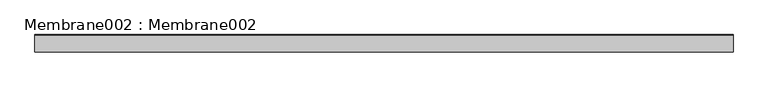
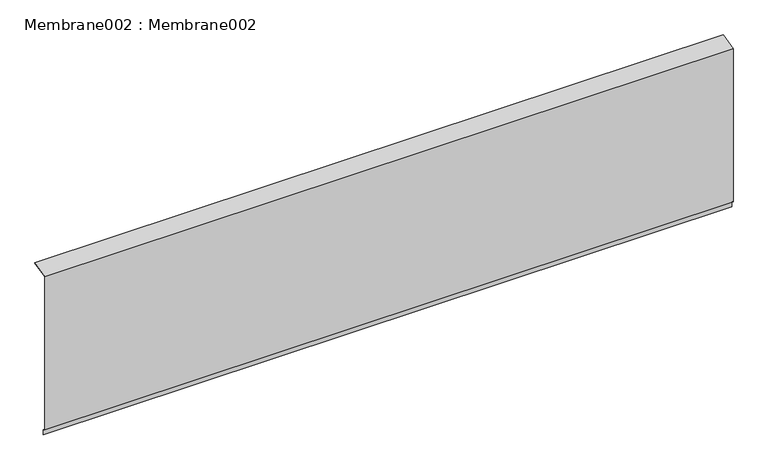
"""IFC4 building model written with IfcOpenShell, lengths in millimetres: proxy geometry, Membrane002 : Membrane002."""

from ifc_helpers import new_model, si_unit, frame, origin, place, context, project, spatial, polyline, outline, extrude, source, transform, mapped, element, save


def membrane002_membrane002_5acc3b50(model_context):
    return source(origin(), model_context, "Body", "SweptSolid", [
        extrude(outline(polyline([(10487.9371885, 43422.3848589), (10439.3258229, 43410.2922698), (10439.3258229, 42942.6633437), (10446.7216797, 42936.3899062), (10446.7216797, 42922.2460937), (10445.2216797, 42922.2460937), (10445.2216797, 42935.6953125), (10437.8258229, 42941.96875), (10437.8258229, 43411.4648437), (10487.5750834, 43423.8404962), (10487.9371885, 43422.3848589)])), frame((3694.2883192, 0.0, 0.0), z_axis=(1.0, 0.0, 0.0), x_axis=(0.0, 1.0, 0.0)), (0.0, 0.0, 1.0), 2000.0),
    ])


if __name__ == "__main__":
    model = new_model("IFC4")
    model_context = context("Model", 3, world=origin())
    ifc_project = project(units=[si_unit("LENGTHUNIT", "METRE", prefix="MILLI")], contexts=[model_context])
    site = spatial("IfcSite", under=ifc_project)
    building = spatial("IfcBuilding", under=site)
    placement = place(None, origin())
    membrane002_membrane002_shape = membrane002_membrane002_5acc3b50(model_context)
    element("IfcBuildingElementProxy", 1, Name="Membrane002 : Membrane002", ObjectType="Membrane002 : Membrane002", at=placement, inside=building, context=model_context, shape_type="MappedRepresentation", body=[
        mapped(membrane002_membrane002_shape, transform((0.0, 0.0, 0.0), x_axis=(1.0, 0.0, 0.0), y_axis=(0.0, 1.0, 0.0), z_axis=(0.0, 0.0, 1.0))),
    ])
    save(model, "model.ifc")

# Revit data of these elements
# Type "Membrane002 : Membrane002"
#   NameOverride = "Membrane002"
# Element 1 (IfcBuildingElementProxy, "Membrane002 : Membrane002")
#   Materials on its faces: "(2) LAYERS OF ICE & WATER SHIELD (BITUTHANE) UNDER STUCCO"
# Materials
#   "(2) LAYERS OF ICE & WATER SHIELD (BITUTHANE) UNDER STUCCO": class "Unassigned", colour RGB 186 255 159, transparency 0, Cost = 0
